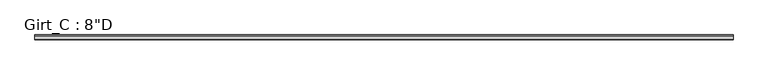
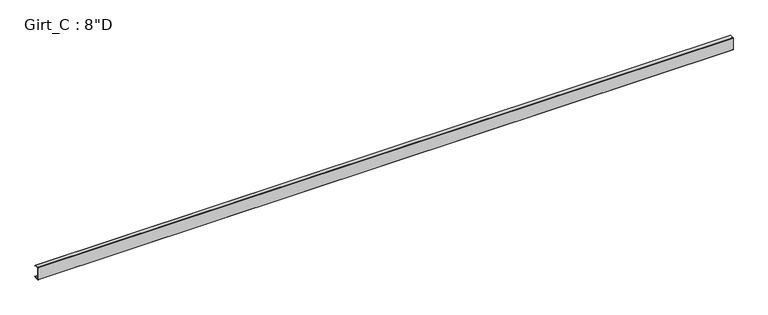
"""IFC4 building model written with IfcOpenShell, lengths in millimetres: beam geometry."""

from ifc_helpers import new_model, si_unit, point, frame, frame_2d, origin, place, context, project, spatial, polyline, circle_curve, trimmed, segment, composite_curve, outline, extrude, source, transform, mapped, element, save


def beam_55619ad5(model_context):
    return source(origin(), model_context, "Body", "SweptSolid", [
        extrude(outline(composite_curve([segment(polyline([(63.5, 101.6), (75.745104, 87.0068534), (73.6169367, 85.221109), (62.204539, 98.821875), (3.3005807, 98.821875)]), True, "CONTINUOUS"), segment(trimmed(circle_curve(frame_2d((3.3741066, 96.8381931)), 1.9850441), [point((3.3005807, 98.821875))], [point((1.3890625, 96.8381931))], True, "CARTESIAN"), True, "CONTINUOUS"), segment(polyline([(1.3890625, 96.8381931), (1.3890625, -96.8389339)]), True, "CONTINUOUS"), segment(trimmed(circle_curve(frame_2d((3.3748024, -96.8389339)), 1.9857399), [point((1.3890625, -96.8389339))], [point((3.2694106, -98.821875))], True, "CARTESIAN"), True, "CONTINUOUS"), segment(polyline([(3.2694106, -98.821875), (62.204539, -98.821875), (73.6169367, -85.221109), (75.745104, -87.0068534), (63.5, -101.6), (3.3734375, -101.6)]), True, "CONTINUOUS"), segment(trimmed(circle_curve(frame_2d((3.3734375, -96.8375)), 4.7625), [point((3.3734375, -101.6))], [point((-1.3890625, -96.8375))], False, "CARTESIAN"), True, "CONTINUOUS"), segment(polyline([(-1.3890625, -96.8375), (-1.3890625, 96.8375)]), True, "CONTINUOUS"), segment(trimmed(circle_curve(frame_2d((3.3734375, 96.8375)), 4.7625), [point((-1.3890625, 96.8375))], [point((3.3734375, 101.6))], False, "CARTESIAN"), True, "CONTINUOUS"), segment(polyline([(3.3734375, 101.6), (63.5, 101.6)]), True, "CONTINUOUS")], self_intersect=False)), frame((-5464.175, 0.0, 0.0), z_axis=(1.0, 0.0, 0.0), x_axis=(0.0, 1.0, 0.0)), (0.0, 0.0, 1.0), 10852.15),
    ])


if __name__ == "__main__":
    model = new_model("IFC4")
    model_context = context("Model", 3, world=origin())
    ifc_project = project(units=[si_unit("LENGTHUNIT", "METRE", prefix="MILLI")], contexts=[model_context])
    site = spatial("IfcSite", under=ifc_project)
    building = spatial("IfcBuilding", under=site)
    placement = place(None, origin())
    beam_shape = beam_55619ad5(model_context)
    element("IfcBeam", 1, ObjectType="Girt_C : 8\"D", at=placement, inside=building, context=model_context, shape_type="MappedRepresentation", body=[
        mapped(beam_shape, transform((0.0, 0.0, 0.0), x_axis=(1.0, 0.0, 0.0), y_axis=(0.0, 1.0, 0.0), z_axis=(0.0, 0.0, 1.0))),
    ])
    save(model, "model.ifc")

# Revit data of these elements
# Type "Girt_C : 8\"D"
#   Web_Thickness = 0' - 0 7/64"
#   Length [instance default] = 10' - 0"
#   Leg_1 = 0' - 2 1/2"
#   Height = 0' - 8"
#   Structural Material [instance default] = none
